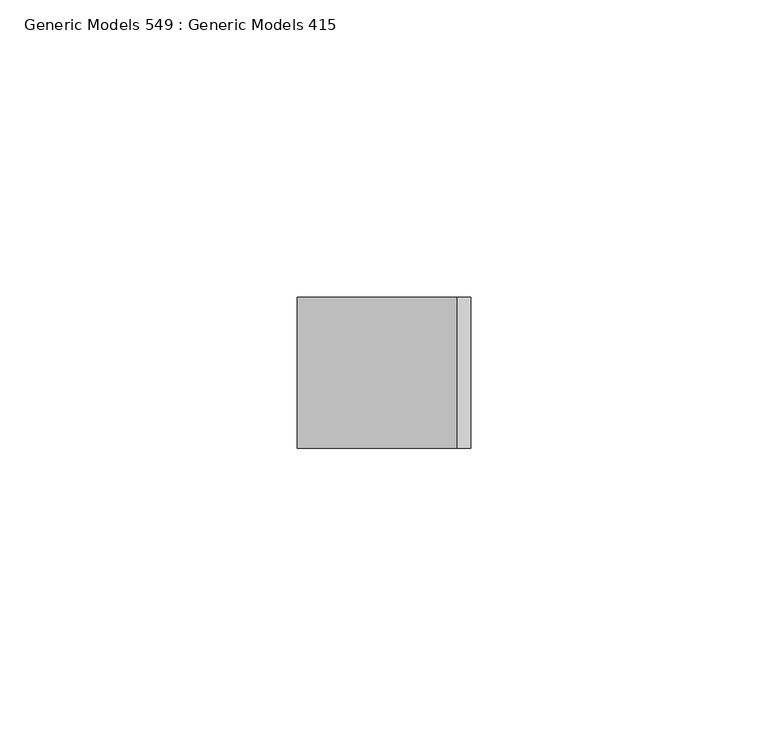
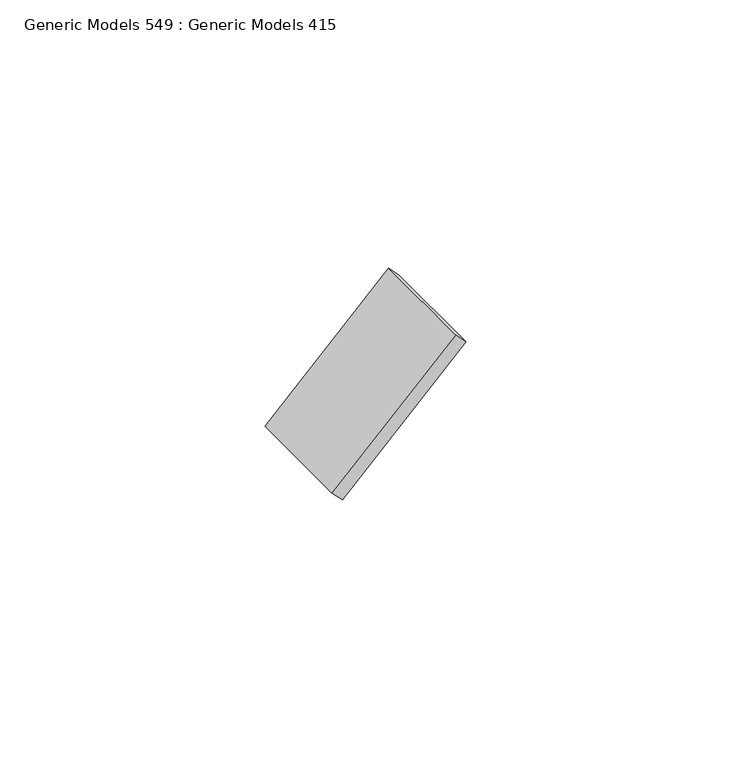
"""IFC4 building model written with IfcOpenShell, lengths in millimetres: proxy geometry, Generic Models 549 : Generic Models 415."""

from ifc_helpers import new_model, si_unit, frame, origin, place, context, project, spatial, polyline, outline, extrude, source, transform, mapped, element, save


def generic_models_549_generic_models_415_feeeb26f(model_context):
    return source(origin(), model_context, "Body", "SweptSolid", [
        extrude(outline(polyline([(0.0, -3.175), (0.0, 0.0), (25.4, 0.0), (25.4, -3.175), (0.0, -3.175)])), frame((7848.0411784, 4501.3863946, 124749.8849742), z_axis=(0.7071067811867181, 0.0, 0.707106781186377), x_axis=(0.0, -1.0, 0.0)), (0.0, 0.0, 1.0), 38.1),
    ])


if __name__ == "__main__":
    model = new_model("IFC4")
    model_context = context("Model", 3, world=origin())
    ifc_project = project(units=[si_unit("LENGTHUNIT", "METRE", prefix="MILLI")], contexts=[model_context])
    site = spatial("IfcSite", under=ifc_project)
    building = spatial("IfcBuilding", under=site)
    placement = place(None, origin())
    generic_models_549_generic_models_415_shape = generic_models_549_generic_models_415_feeeb26f(model_context)
    element("IfcBuildingElementProxy", 1, Name="Generic Models 549 : Generic Models 415", ObjectType="Generic Models 549 : Generic Models 415", at=placement, inside=building, context=model_context, shape_type="MappedRepresentation", body=[
        mapped(generic_models_549_generic_models_415_shape, transform((0.0, 0.0, 0.0), x_axis=(1.0, 0.0, 0.0), y_axis=(0.0, 1.0, 0.0), z_axis=(0.0, 0.0, 1.0))),
    ])
    save(model, "model.ifc")

# Revit data of these elements
# Element 1 (IfcBuildingElementProxy, "Generic Models 549 : Generic Models 415")
#   Materials on its faces: "_WELDED STEEL TABS FOR LOUVER ATTACHMENT"
# Materials
#   "_WELDED STEEL TABS FOR LOUVER ATTACHMENT": class "Metal", colour RGB 199 199 199, transparency 0, Description = "Structural steel 50ksi", Cost = 0
